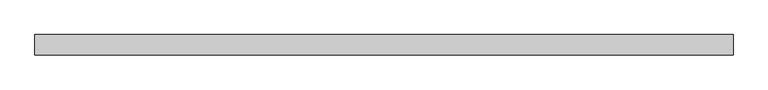
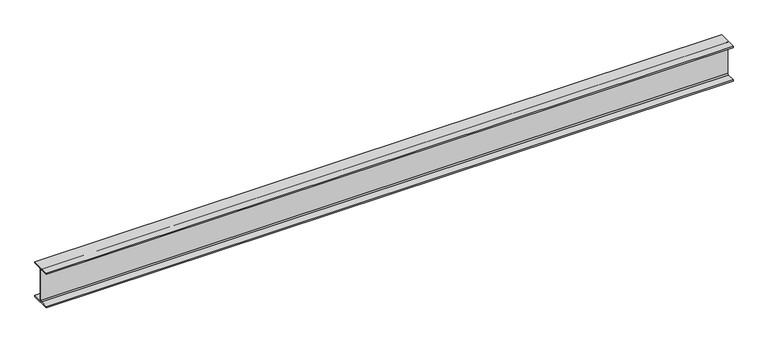
"""IFC4 building model written with IfcOpenShell, lengths in millimetres: beam geometry, Old_Steel Beam_H-KSD3502 : H_SB_ASB_H-340×250x9x14."""

from ifc_helpers import new_model, si_unit, point, frame, frame_2d, origin, place, context, project, spatial, polyline, circle_curve, trimmed, segment, composite_curve, outline, extrude, source, transform, mapped, element, save


def beam_497e65e0(model_context):
    return source(origin(), model_context, "Body", "SweptSolid", [
        extrude(outline(composite_curve([segment(polyline([(82.5, -141.5), (82.5, -151.7), (-82.5, -151.7), (-82.5, -141.5), (-11.9, -141.5)]), True, "CONTINUOUS"), segment(trimmed(circle_curve(frame_2d((-11.9, -132.6)), 8.9), [point((-11.9, -141.5))], [point((-3.0, -132.6))], True, "CARTESIAN"), True, "CONTINUOUS"), segment(polyline([(-3.0, -132.6), (-3.0, 132.6)]), True, "CONTINUOUS"), segment(trimmed(circle_curve(frame_2d((-11.9, 132.6)), 8.9), [point((-3.0, 132.6))], [point((-11.9, 141.5))], True, "CARTESIAN"), True, "CONTINUOUS"), segment(polyline([(-11.9, 141.5), (-82.5, 141.5), (-82.5, 151.7), (82.5, 151.7), (82.5, 141.5), (11.9, 141.5)]), True, "CONTINUOUS"), segment(trimmed(circle_curve(frame_2d((11.9, 132.6)), 8.9), [point((11.9, 141.5))], [point((3.0, 132.6))], True, "CARTESIAN"), True, "CONTINUOUS"), segment(polyline([(3.0, 132.6), (3.0, -132.6)]), True, "CONTINUOUS"), segment(trimmed(circle_curve(frame_2d((11.9, -132.6)), 8.9), [point((3.0, -132.6))], [point((11.9, -141.5))], True, "CARTESIAN"), True, "CONTINUOUS"), segment(polyline([(11.9, -141.5), (82.5, -141.5)]), True, "CONTINUOUS")], self_intersect=False)), frame((-2837.3, 0.0, 0.0), z_axis=(1.0, 0.0, 0.0), x_axis=(0.0, 1.0, 0.0)), (0.0, 0.0, 1.0), 5674.6),
    ])


if __name__ == "__main__":
    model = new_model("IFC4")
    model_context = context("Model", 3, world=origin())
    ifc_project = project(units=[si_unit("LENGTHUNIT", "METRE", prefix="MILLI")], contexts=[model_context])
    site = spatial("IfcSite", under=ifc_project)
    building = spatial("IfcBuilding", under=site)
    placement = place(None, origin())
    beam_shape = beam_497e65e0(model_context)
    element("IfcBeam", 1, ObjectType="Old_Steel Beam_H-KSD3502 : H_SB_ASB_H-340×250x9x14", at=placement, inside=building, context=model_context, shape_type="MappedRepresentation", body=[
        mapped(beam_shape, transform((0.0, 0.0, 0.0), x_axis=(1.0, 0.0, 0.0), y_axis=(0.0, 1.0, 0.0), z_axis=(0.0, 0.0, 1.0))),
    ])
    save(model, "model.ifc")

# Revit data of these elements
# Type "Old_Steel Beam_H-KSD3502 : H_SB_ASB_H-340×250x9x14"
#   Width = 25.0 cm
#   Web Thickness = 0.9 cm
#   Web Fillet = 2.0 cm
#   Warping Constant = 968661.0 cm⁶
#   Torsional Moment of Inertia = 53.6551 cm⁴
#   Torsional Modulus = 1.0 cm³
#   Section Area = 101.5 cm²
#   Plastic Modulus weak axis = 447.0 cm³
#   Plastic Modulus strong axis = 1410.0 cm³
#   Perimeter = 1.63 m²/m
#   Nominal Weight = 79.70 kgf/m
#   Moment of Inertia weak axis = 3650.00 cm⁴
#   Moment of Inertia strong axis = 21700.00 cm⁴
#   Height = 34.0 cm
#   Flange Thickness = 1.4 cm
#   Elastic Modulus weak axis = 292.0 cm³
#   Elastic Modulus strong axis = 1280.0 cm³
#   Centroid Vertical = 17.0 cm
#   Centroid Horizontal = 12.5 cm
#   Length [instance default] = 1.5240 m
#   Structural Material [instance default] = Steel, 45-345
#   Assembly Code = ""
# Element 1 (IfcBeam, "Old_Steel Beam_H-KSD3502 : H_SB_ASB_H-340×250x9x14")
#   Structural Material = none
# Materials
#   "Steel, 45-345": class "Metal", colour RGB 189 187 185, transparency 0, Description = "Steel 345 MPa", Cost = 0
